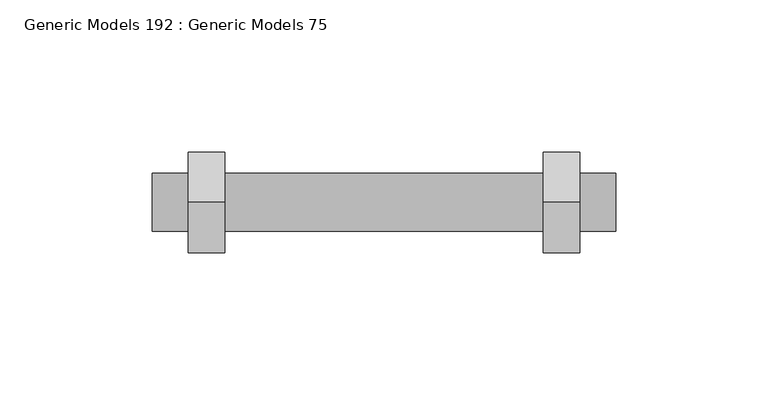
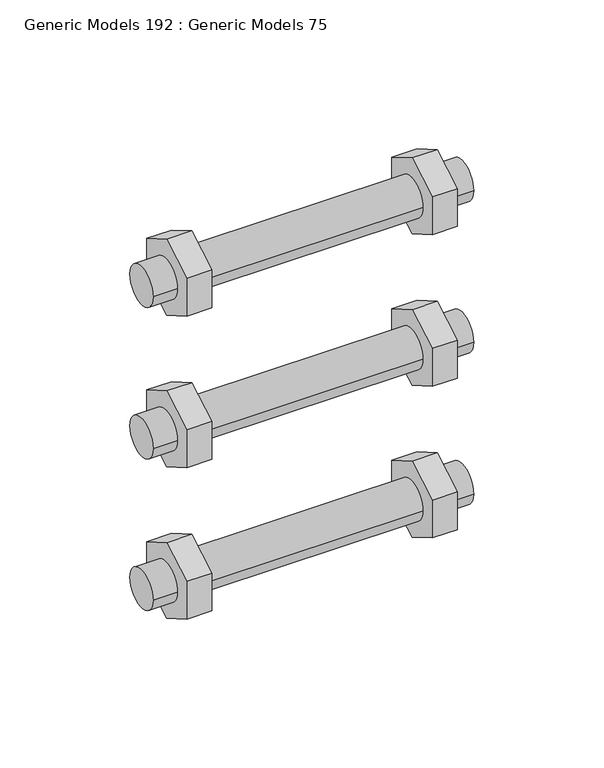
"""IFC4 building model written with IfcOpenShell, lengths in millimetres: proxy geometry, Generic Models 192 : Generic Models 75."""

from ifc_helpers import new_model, si_unit, point, frame, frame_2d, origin, place, context, project, spatial, polyline, circle_curve, trimmed, segment, composite_curve, outline, extrude, source, transform, mapped, element, save


def generic_models_192_generic_models_75_29abc1e5(model_context):
    return source(origin(), model_context, "Body", "SweptSolid", [
        extrude(outline(polyline([(35428.1042603, 269062.859622), (35444.6020442, 269072.384622), (35461.0998281, 269062.859622), (35461.0998281, 269043.809622), (35444.6020442, 269034.284622), (35428.1042603, 269043.809622), (35428.1042603, 269062.859622)])), frame((31918.2596032, 0.0, 0.0), z_axis=(1.0, 0.0, 0.0), x_axis=(0.0, 1.0, 0.0)), (0.0, 0.0, 1.0), 11.90625),
        extrude(outline(polyline([(35428.1042603, 268986.659622), (35444.6020442, 268996.184622), (35461.0998281, 268986.659622), (35461.0998281, 268967.609622), (35444.6020442, 268958.084622), (35428.1042603, 268967.609622), (35428.1042603, 268986.659622)])), frame((31918.2596032, 0.0, 0.0), z_axis=(1.0, 0.0, 0.0), x_axis=(0.0, 1.0, 0.0)), (0.0, 0.0, 1.0), 11.90625),
        extrude(outline(polyline([(35428.1042603, 268910.459622), (35444.6020442, 268919.984622), (35461.0998281, 268910.459622), (35461.0998281, 268891.409622), (35444.6020442, 268881.884622), (35428.1042603, 268891.409622), (35428.1042603, 268910.459622)])), frame((31918.2596032, 0.0, 0.0), z_axis=(1.0, 0.0, 0.0), x_axis=(0.0, 1.0, 0.0)), (0.0, 0.0, 1.0), 11.90625),
        extrude(outline(polyline([(35428.1042603, 269062.859622), (35444.6020442, 269072.384622), (35461.0998281, 269062.859622), (35461.0998281, 269043.809622), (35444.6020442, 269034.284622), (35428.1042603, 269043.809622), (35428.1042603, 269062.859622)])), frame((31801.5783532, 0.0, 0.0), z_axis=(1.0, 0.0, 0.0), x_axis=(0.0, 1.0, 0.0)), (0.0, 0.0, 1.0), 11.90625),
        extrude(outline(polyline([(35428.1042603, 268986.659622), (35444.6020442, 268996.184622), (35461.0998281, 268986.659622), (35461.0998281, 268967.609622), (35444.6020442, 268958.084622), (35428.1042603, 268967.609622), (35428.1042603, 268986.659622)])), frame((31801.5783532, 0.0, 0.0), z_axis=(1.0, 0.0, 0.0), x_axis=(0.0, 1.0, 0.0)), (0.0, 0.0, 1.0), 11.90625),
        extrude(outline(polyline([(35428.1042603, 268910.459622), (35444.6020442, 268919.984622), (35461.0998281, 268910.459622), (35461.0998281, 268891.409622), (35444.6020442, 268881.884622), (35428.1042603, 268891.409622), (35428.1042603, 268910.459622)])), frame((31801.5783532, 0.0, 0.0), z_axis=(1.0, 0.0, 0.0), x_axis=(0.0, 1.0, 0.0)), (0.0, 0.0, 1.0), 11.90625),
        extrude(outline(composite_curve([segment(trimmed(circle_curve(frame_2d((35444.6020442, 268977.134622)), 9.525), [point((35454.1270442, 268977.134622))], [point((35435.0770442, 268977.134622))], False, "CARTESIAN"), True, "CONTINUOUS"), segment(trimmed(circle_curve(frame_2d((35444.6020442, 268977.134622)), 9.525), [point((35435.0770442, 268977.134622))], [point((35454.1270442, 268977.134622))], False, "CARTESIAN"), True, "CONTINUOUS")], self_intersect=False)), frame((31789.6721032, 0.0, 0.0), z_axis=(1.0, 0.0, 0.0), x_axis=(0.0, 1.0, 0.0)), (0.0, 0.0, 1.0), 152.4),
        extrude(outline(composite_curve([segment(trimmed(circle_curve(frame_2d((35444.6020442, 268900.934622)), 9.525), [point((35454.1270442, 268900.934622))], [point((35435.0770442, 268900.934622))], False, "CARTESIAN"), True, "CONTINUOUS"), segment(trimmed(circle_curve(frame_2d((35444.6020442, 268900.934622)), 9.525), [point((35435.0770442, 268900.934622))], [point((35454.1270442, 268900.934622))], False, "CARTESIAN"), True, "CONTINUOUS")], self_intersect=False)), frame((31789.6721032, 0.0, 0.0), z_axis=(1.0, 0.0, 0.0), x_axis=(0.0, 1.0, 0.0)), (0.0, 0.0, 1.0), 152.4),
        extrude(outline(composite_curve([segment(trimmed(circle_curve(frame_2d((35444.6020442, 269053.334622)), 9.525), [point((35454.1270442, 269053.334622))], [point((35435.0770442, 269053.334622))], False, "CARTESIAN"), True, "CONTINUOUS"), segment(trimmed(circle_curve(frame_2d((35444.6020442, 269053.334622)), 9.525), [point((35435.0770442, 269053.334622))], [point((35454.1270442, 269053.334622))], False, "CARTESIAN"), True, "CONTINUOUS")], self_intersect=False)), frame((31789.6721032, 0.0, 0.0), z_axis=(1.0, 0.0, 0.0), x_axis=(0.0, 1.0, 0.0)), (0.0, 0.0, 1.0), 152.4),
    ])


if __name__ == "__main__":
    model = new_model("IFC4")
    model_context = context("Model", 3, world=origin())
    ifc_project = project(units=[si_unit("LENGTHUNIT", "METRE", prefix="MILLI")], contexts=[model_context])
    site = spatial("IfcSite", under=ifc_project)
    building = spatial("IfcBuilding", under=site)
    placement = place(None, origin())
    generic_models_192_generic_models_75_shape = generic_models_192_generic_models_75_29abc1e5(model_context)
    element("IfcBuildingElementProxy", 1, Name="Generic Models 192 : Generic Models 75", ObjectType="Generic Models 192 : Generic Models 75", at=placement, inside=building, context=model_context, shape_type="MappedRepresentation", body=[
        mapped(generic_models_192_generic_models_75_shape, transform((0.0, 0.0, 0.0), x_axis=(1.0, 0.0, 0.0), y_axis=(0.0, 1.0, 0.0), z_axis=(0.0, 0.0, 1.0))),
    ])
    save(model, "model.ifc")
